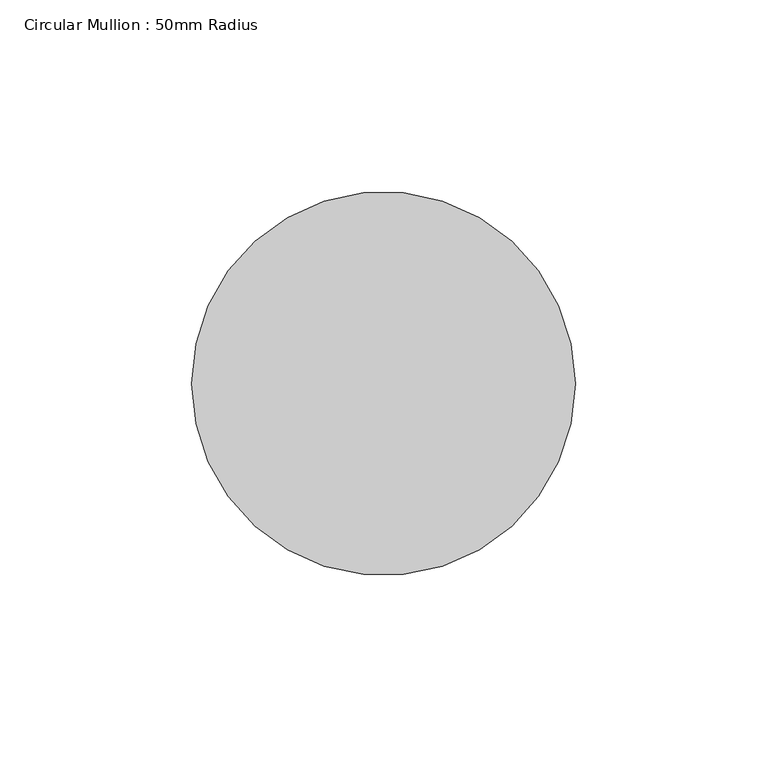
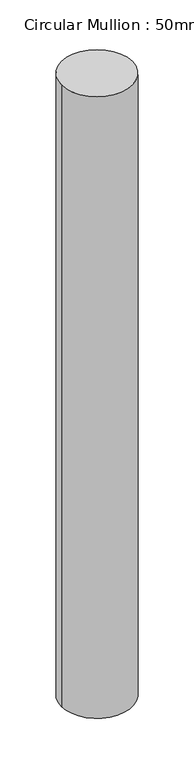
"""IFC4 building model written with IfcOpenShell, lengths in millimetres: member geometry, Circular Mullion : 50mm Radius."""

from ifc_helpers import new_model, si_unit, point, frame, origin, origin_2d, place, context, project, spatial, circle_curve, trimmed, segment, composite_curve, outline, extrude, source, transform, mapped, element, save


def circular_mullion_50mm_radius_9692996e(model_context):
    return source(origin(), model_context, "Body", "SweptSolid", [
        extrude(outline(composite_curve([segment(trimmed(circle_curve(origin_2d(), 50.0), [point((50.0, 0.0))], [point((-50.0, 0.0))], False, "CARTESIAN"), True, "CONTINUOUS"), segment(trimmed(circle_curve(origin_2d(), 50.0), [point((-50.0, 0.0))], [point((50.0, 0.0))], False, "CARTESIAN"), True, "CONTINUOUS")], self_intersect=False)), frame((0.0, 0.0, -924.4330076), z_axis=(0.0, 0.0, 1.0), x_axis=(1.0, 0.0, 0.0)), (0.0, 0.0, 1.0), 924.4330076),
    ])


if __name__ == "__main__":
    model = new_model("IFC4")
    model_context = context("Model", 3, world=origin())
    ifc_project = project(units=[si_unit("LENGTHUNIT", "METRE", prefix="MILLI")], contexts=[model_context])
    site = spatial("IfcSite", under=ifc_project)
    building = spatial("IfcBuilding", under=site)
    placement = place(None, origin())
    circular_mullion_50mm_radius_shape = circular_mullion_50mm_radius_9692996e(model_context)
    element("IfcMember", 1, ObjectType="Circular Mullion : 50mm Radius", at=placement, inside=building, context=model_context, shape_type="MappedRepresentation", body=[
        mapped(circular_mullion_50mm_radius_shape, transform((0.0, 0.0, 0.0), x_axis=(1.0, 0.0, 0.0), y_axis=(0.0, 1.0, 0.0), z_axis=(0.0, 0.0, 1.0))),
    ])
    save(model, "model.ifc")

# Revit data of these elements
# Type "Circular Mullion : 50mm Radius"
#   built-in parameter 1007350 = 0.164042 (stored number, unit not read)
# Element 1 (IfcMember, "Circular Mullion : 50mm Radius")
#   Materials on its faces: "Aluminium"
# Materials
#   "Aluminium": class "Metal", colour RGB 247 247 247, transparency 0, Description = "Aluminium 6061", Cost = 0
